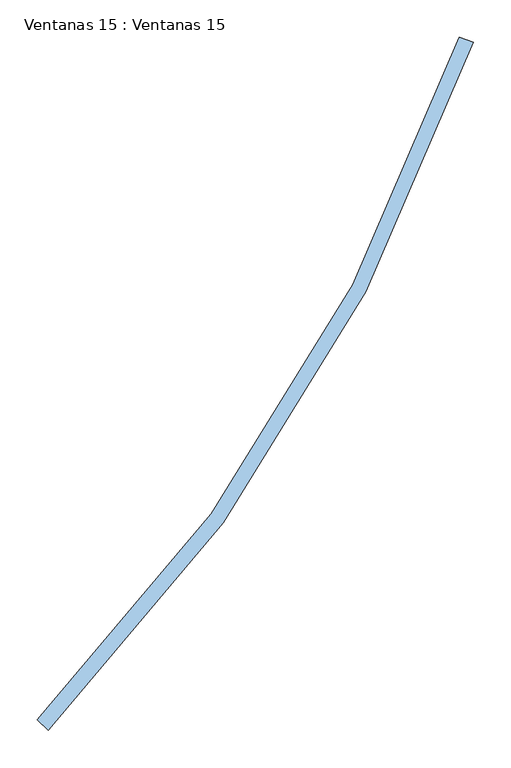
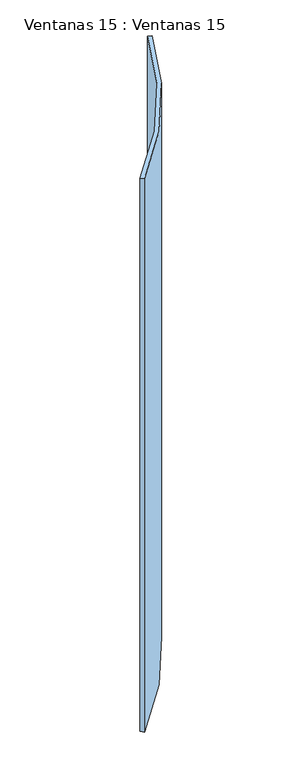
"""IFC4 building model written with IfcOpenShell, lengths in millimetres: window geometry, Ventanas 15 : Ventanas 15."""

from ifc_helpers import new_model, si_unit, point, frame, frame_2d, origin, place, context, project, spatial, polyline, circle_curve, trimmed, segment, composite_curve, outline, extrude, source, transform, mapped, element, save


def ventanas_15_ventanas_15_15e3fe58(model_context):
    return source(origin(), model_context, "Body", "SweptSolid", [
        extrude(outline(composite_curve([segment(polyline([(-4390.4724617, -4829.0440235), (-4404.6145974, -4814.9018879)]), True, "CONTINUOUS"), segment(trimmed(circle_curve(frame_2d((-6149.5179321, -3107.4095296)), 2441.3557302), [point((-4404.6145974, -4814.9018879))], [point((-3842.2330689, -3905.3157654))], True, "CARTESIAN"), True, "CONTINUOUS"), segment(polyline([(-3842.2330689, -3905.3157654), (-3823.3313931, -3911.852328)]), True, "CONTINUOUS"), segment(trimmed(circle_curve(frame_2d((-6149.4961438, -3107.4198771)), 2461.3317565), [point((-3823.3313931, -3911.852328))], [point((-4390.4724617, -4829.0440235))], False, "CARTESIAN"), True, "CONTINUOUS")], self_intersect=False)), frame((0.0, 0.0, 6100.0), z_axis=(0.0, 0.0, 1.0), x_axis=(1.0, 0.0, 0.0)), (0.0, 0.0, 1.0), 2919.1210755),
    ])


if __name__ == "__main__":
    model = new_model("IFC4")
    model_context = context("Model", 3, world=origin())
    ifc_project = project(units=[si_unit("LENGTHUNIT", "METRE", prefix="MILLI")], contexts=[model_context])
    site = spatial("IfcSite", under=ifc_project)
    building = spatial("IfcBuilding", under=site)
    placement = place(None, origin())
    ventanas_15_ventanas_15_shape = ventanas_15_ventanas_15_15e3fe58(model_context)
    element("IfcWindow", 1, ObjectType="Ventanas 15 : Ventanas 15", at=placement, inside=building, context=model_context, shape_type="MappedRepresentation", body=[
        mapped(ventanas_15_ventanas_15_shape, transform((0.0, 0.0, 0.0), x_axis=(1.0, 0.0, 0.0), y_axis=(0.0, 1.0, 0.0), z_axis=(0.0, 0.0, 1.0))),
    ])
    save(model, "model.ifc")

# Revit data of these elements
# Project information
#   Fecha de emisión de proyecto = "29 de Mayo de 2020"
#   Estado de proyecto = "Project  Status"
#   Nombre de cliente = "Ariel Herbst"
#   Dirección de proyecto = "## Street\nCity, State  Zip"
#   Nombre de proyecto = "Seminario II"
#   Número de proyecto = "0001"
# Type "Ventanas 15 : Ventanas 15"
#   Type Mark = "41"
# Element 1 (IfcWindow, "Ventanas 15 : Ventanas 15")
#   Materials on its faces: "VIDRIO"
# Materials
#   "VIDRIO": class "Genérico", colour RGB 120 120 120, transparency 0, Cost = 0
